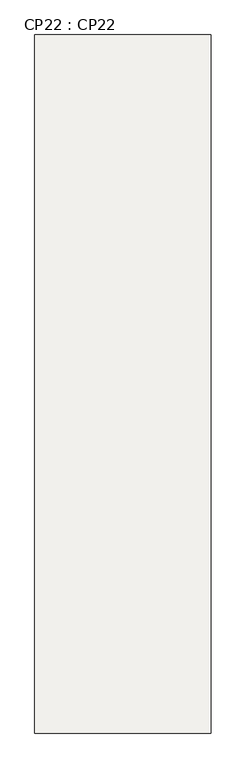
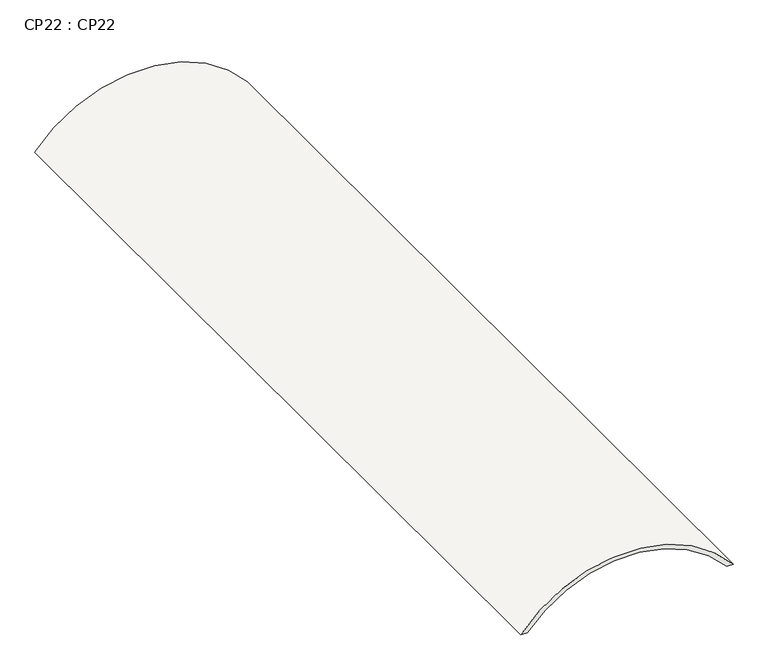
"""IFC4 building model written with IfcOpenShell, lengths in millimetres: slab geometry, CP22 : CP22."""

from ifc_helpers import new_model, si_unit, point, frame, frame_2d, origin, place, context, project, spatial, polyline, circle_curve, trimmed, segment, composite_curve, outline, extrude, source, transform, mapped, element, save


def cp22_cp22_92024077(model_context):
    return source(origin(), model_context, "Body", "SweptSolid", [
        extrude(outline(composite_curve([segment(trimmed(circle_curve(frame_2d((12562.2036417, 42833.2245513)), 3237.981756), [point((14620.0, 45333.2245512))], [point((14620.0, 40333.2245513))], False, "CARTESIAN"), True, "CONTINUOUS"), segment(polyline([(14620.0, 40333.2245513), (14620.0, 40483.2245513)]), True, "CONTINUOUS"), segment(trimmed(circle_curve(frame_2d((12603.8185575, 42833.2245513)), 3096.3668402), [point((14620.0, 40483.2245513))], [point((14620.0, 45183.2245512))], True, "CARTESIAN"), True, "CONTINUOUS"), segment(polyline([(14620.0, 45183.2245512), (14620.0, 45333.2245512)]), True, "CONTINUOUS")], self_intersect=False)), frame((0.0, -100.2551788, 0.0), z_axis=(0.0, 1.0, 0.0), x_axis=(0.0, 0.0, 1.0)), (0.0, 0.0, 1.0), 19800.2551781),
    ])


if __name__ == "__main__":
    model = new_model("IFC4")
    model_context = context("Model", 3, world=origin())
    ifc_project = project(units=[si_unit("LENGTHUNIT", "METRE", prefix="MILLI")], contexts=[model_context])
    site = spatial("IfcSite", under=ifc_project)
    building = spatial("IfcBuilding", under=site)
    placement = place(None, origin())
    cp22_cp22_shape = cp22_cp22_92024077(model_context)
    element("IfcSlab", 1, ObjectType="CP22 : CP22", at=placement, inside=building, context=model_context, shape_type="MappedRepresentation", body=[
        mapped(cp22_cp22_shape, transform((0.0, 0.0, 0.0), x_axis=(1.0, 0.0, 0.0), y_axis=(0.0, 1.0, 0.0), z_axis=(0.0, 0.0, 1.0))),
    ])
    save(model, "model.ifc")

# Revit data of these elements
# Element 1 (IfcSlab, "CP22 : CP22")
#   Materials on its faces: "Concrete, RC"
# Materials
#   "Concrete, RC": class "Concrete", colour RGB 128 128 128, transparency 0, Description = "Cast-in-place concrete", Cost = 0
